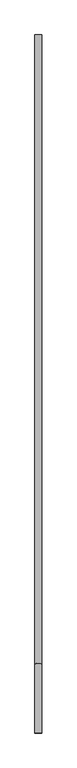
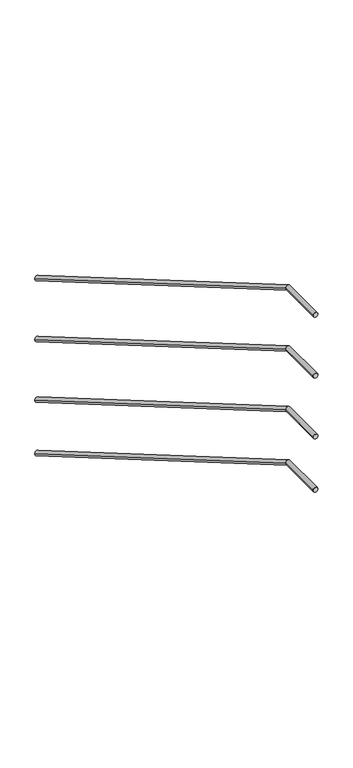
"""IFC4 building model written with IfcOpenShell, lengths in millimetres: railing geometry."""

from ifc_helpers import new_model, si_unit, frame, origin, place, context, project, spatial, circle_curve, ellipse_curve, source, transform, mapped, element, save
from ifc_brep_helpers import plane_surface, cylinder_surface, advanced_brep


def railing_58bcc5ab(model_context):
    return source(origin(), model_context, "Body", "AdvancedBrep", [
        advanced_brep(
        [(-1709.6, 15799.5208589, 8657.5963084), (-1739.6, 15799.5208589, 8657.5963084), (-1709.6, 13095.4656218, 10234.9618634), (-1739.6, 13095.4656218, 10234.9618634), (-1709.6, 12799.5208589, 10234.9618634), (-1739.6, 12799.5208589, 10234.9618634)],
        [
            (0, 1, ellipse_curve(frame((-1724.6, 15799.5208589, 8657.5963084), z_axis=(0.0, 1.0, 0.0), x_axis=(0.0, 0.0, -1.0)), 17.365555, 15.0)),
            (1, 0, ellipse_curve(frame((-1724.6, 15799.5208589, 8657.5963084), z_axis=(0.0, 1.0, 0.0), x_axis=(0.0, 0.0, -1.0)), 17.365555, 15.0)),
            (0, 2),
            (2, 3, ellipse_curve(frame((-1724.6, 13095.4656218, 10234.9618634), z_axis=(0.0, 0.9653442134540492, -0.2609799792144661), x_axis=(0.0, -0.26097997921446625, -0.9653442134540491)), 15.5384989, 15.0)),
            (3, 1),
            (3, 2, ellipse_curve(frame((-1724.6, 13095.4656218, 10234.9618634), z_axis=(0.0, 0.9653442134540492, -0.2609799792144661), x_axis=(0.0, -0.26097997921446625, -0.9653442134540491)), 15.5384989, 15.0)),
            (4, 5, circle_curve(frame((-1724.6, 12799.5208589, 10234.9618634), z_axis=(0.0, -1.0, 0.0), x_axis=(-1.0, 0.0, 0.0)), 15.0)),
            (5, 4, circle_curve(frame((-1724.6, 12799.5208589, 10234.9618634), z_axis=(0.0, -1.0, 0.0), x_axis=(-1.0, 0.0, 0.0)), 15.0)),
            (2, 4),
            (5, 3),
        ],
        [
            plane_surface(frame((-1724.6, 15799.5208589, 8674.9618634), z_axis=(0.0, 1.0, 0.0), x_axis=(0.0, 0.0, -1.0))),
            cylinder_surface(frame((-1724.6, 15791.9627935, 8662.0051799), z_axis=(0.0, 0.8637789008984337, -0.5038710255240858), x_axis=(-1.0, 0.0, 0.0)), 15.0),
            plane_surface(frame((-1724.6, 12799.5208589, 10249.9618634), z_axis=(0.0, -1.0, 0.0), x_axis=(0.0, 0.0, -1.0))),
            cylinder_surface(frame((-1724.6, 13099.5208589, 10234.9618634), z_axis=(0.0, 1.0, 0.0), x_axis=(-1.0, 0.0, 0.0)), 15.0),
        ],
        [
            (0, [[1, 2]]),
            (1, [[-1, 3, 4, 5]]),
            (1, [[-2, -5, 6, -3]]),
            (2, [[7, 8]]),
            (3, [[-4, 9, -8, 10]]),
            (3, [[-6, -10, -7, -9]]),
        ],
    ),
        advanced_brep(
        [(-1709.6, 15799.5208589, 7857.5963084), (-1739.6, 15799.5208589, 7857.5963084), (-1709.6, 13095.4656218, 9434.9618634), (-1739.6, 13095.4656218, 9434.9618634), (-1709.6, 12799.5208589, 9434.9618634), (-1739.6, 12799.5208589, 9434.9618634)],
        [
            (0, 1, ellipse_curve(frame((-1724.6, 15799.5208589, 7857.5963084), z_axis=(0.0, 1.0, 0.0), x_axis=(0.0, 0.0, -1.0)), 17.365555, 15.0)),
            (1, 0, ellipse_curve(frame((-1724.6, 15799.5208589, 7857.5963084), z_axis=(0.0, 1.0, 0.0), x_axis=(0.0, 0.0, -1.0)), 17.365555, 15.0)),
            (0, 2),
            (2, 3, ellipse_curve(frame((-1724.6, 13095.4656218, 9434.9618634), z_axis=(0.0, 0.9653442134540492, -0.2609799792144661), x_axis=(0.0, -0.26097997921446625, -0.9653442134540491)), 15.5384989, 15.0)),
            (3, 1),
            (3, 2, ellipse_curve(frame((-1724.6, 13095.4656218, 9434.9618634), z_axis=(0.0, 0.9653442134540492, -0.2609799792144661), x_axis=(0.0, -0.26097997921446625, -0.9653442134540491)), 15.5384989, 15.0)),
            (4, 5, circle_curve(frame((-1724.6, 12799.5208589, 9434.9618634), z_axis=(0.0, -1.0, 0.0), x_axis=(-1.0, 0.0, 0.0)), 15.0)),
            (5, 4, circle_curve(frame((-1724.6, 12799.5208589, 9434.9618634), z_axis=(0.0, -1.0, 0.0), x_axis=(-1.0, 0.0, 0.0)), 15.0)),
            (2, 4),
            (5, 3),
        ],
        [
            plane_surface(frame((-1724.6, 15799.5208589, 7874.9618634), z_axis=(0.0, 1.0, 0.0), x_axis=(0.0, 0.0, -1.0))),
            cylinder_surface(frame((-1724.6, 15791.9627935, 7862.0051799), z_axis=(0.0, 0.8637789008984337, -0.5038710255240858), x_axis=(-1.0, 0.0, 0.0)), 15.0),
            plane_surface(frame((-1724.6, 12799.5208589, 9449.9618634), z_axis=(0.0, -1.0, 0.0), x_axis=(0.0, 0.0, -1.0))),
            cylinder_surface(frame((-1724.6, 13099.5208589, 9434.9618634), z_axis=(0.0, 1.0, 0.0), x_axis=(-1.0, 0.0, 0.0)), 15.0),
        ],
        [
            (0, [[1, 2]]),
            (1, [[-1, 3, 4, 5]]),
            (1, [[-2, -5, 6, -3]]),
            (2, [[7, 8]]),
            (3, [[-4, 9, -8, 10]]),
            (3, [[-6, -10, -7, -9]]),
        ],
    ),
        advanced_brep(
        [(-1709.6, 15799.5208589, 8257.5963084), (-1739.6, 15799.5208589, 8257.5963084), (-1709.6, 13095.4656218, 9834.9618634), (-1739.6, 13095.4656218, 9834.9618634), (-1709.6, 12799.5208589, 9834.9618634), (-1739.6, 12799.5208589, 9834.9618634)],
        [
            (0, 1, ellipse_curve(frame((-1724.6, 15799.5208589, 8257.5963084), z_axis=(0.0, 1.0, 0.0), x_axis=(0.0, 0.0, -1.0)), 17.365555, 15.0)),
            (1, 0, ellipse_curve(frame((-1724.6, 15799.5208589, 8257.5963084), z_axis=(0.0, 1.0, 0.0), x_axis=(0.0, 0.0, -1.0)), 17.365555, 15.0)),
            (0, 2),
            (2, 3, ellipse_curve(frame((-1724.6, 13095.4656218, 9834.9618634), z_axis=(0.0, 0.9653442134540492, -0.2609799792144661), x_axis=(0.0, -0.26097997921446625, -0.9653442134540491)), 15.5384989, 15.0)),
            (3, 1),
            (3, 2, ellipse_curve(frame((-1724.6, 13095.4656218, 9834.9618634), z_axis=(0.0, 0.9653442134540492, -0.2609799792144661), x_axis=(0.0, -0.26097997921446625, -0.9653442134540491)), 15.5384989, 15.0)),
            (4, 5, circle_curve(frame((-1724.6, 12799.5208589, 9834.9618634), z_axis=(0.0, -1.0, 0.0), x_axis=(-1.0, 0.0, 0.0)), 15.0)),
            (5, 4, circle_curve(frame((-1724.6, 12799.5208589, 9834.9618634), z_axis=(0.0, -1.0, 0.0), x_axis=(-1.0, 0.0, 0.0)), 15.0)),
            (2, 4),
            (5, 3),
        ],
        [
            plane_surface(frame((-1724.6, 15799.5208589, 8274.9618634), z_axis=(0.0, 1.0, 0.0), x_axis=(0.0, 0.0, -1.0))),
            cylinder_surface(frame((-1724.6, 15791.9627935, 8262.0051799), z_axis=(0.0, 0.8637789008984337, -0.5038710255240858), x_axis=(-1.0, 0.0, 0.0)), 15.0),
            plane_surface(frame((-1724.6, 12799.5208589, 9849.9618634), z_axis=(0.0, -1.0, 0.0), x_axis=(0.0, 0.0, -1.0))),
            cylinder_surface(frame((-1724.6, 13099.5208589, 9834.9618634), z_axis=(0.0, 1.0, 0.0), x_axis=(-1.0, 0.0, 0.0)), 15.0),
        ],
        [
            (0, [[1, 2]]),
            (1, [[-1, 3, 4, 5]]),
            (1, [[-2, -5, 6, -3]]),
            (2, [[7, 8]]),
            (3, [[-4, 9, -8, 10]]),
            (3, [[-6, -10, -7, -9]]),
        ],
    ),
        advanced_brep(
        [(-1709.6, 15799.5208589, 7507.5963084), (-1739.6, 15799.5208589, 7507.5963084), (-1709.6, 13095.4656218, 9084.9618634), (-1739.6, 13095.4656218, 9084.9618634), (-1709.6, 12799.5208589, 9084.9618634), (-1739.6, 12799.5208589, 9084.9618634)],
        [
            (0, 1, ellipse_curve(frame((-1724.6, 15799.5208589, 7507.5963084), z_axis=(0.0, 1.0, 0.0), x_axis=(0.0, 0.0, -1.0)), 17.365555, 15.0)),
            (1, 0, ellipse_curve(frame((-1724.6, 15799.5208589, 7507.5963084), z_axis=(0.0, 1.0, 0.0), x_axis=(0.0, 0.0, -1.0)), 17.365555, 15.0)),
            (0, 2),
            (2, 3, ellipse_curve(frame((-1724.6, 13095.4656218, 9084.9618634), z_axis=(0.0, 0.9653442134540492, -0.2609799792144661), x_axis=(0.0, -0.26097997921446625, -0.9653442134540491)), 15.5384989, 15.0)),
            (3, 1),
            (3, 2, ellipse_curve(frame((-1724.6, 13095.4656218, 9084.9618634), z_axis=(0.0, 0.9653442134540492, -0.2609799792144661), x_axis=(0.0, -0.26097997921446625, -0.9653442134540491)), 15.5384989, 15.0)),
            (4, 5, circle_curve(frame((-1724.6, 12799.5208589, 9084.9618634), z_axis=(0.0, -1.0, 0.0), x_axis=(-1.0, 0.0, 0.0)), 15.0)),
            (5, 4, circle_curve(frame((-1724.6, 12799.5208589, 9084.9618634), z_axis=(0.0, -1.0, 0.0), x_axis=(-1.0, 0.0, 0.0)), 15.0)),
            (2, 4),
            (5, 3),
        ],
        [
            plane_surface(frame((-1724.6, 15799.5208589, 7524.9618634), z_axis=(0.0, 1.0, 0.0), x_axis=(0.0, 0.0, -1.0))),
            cylinder_surface(frame((-1724.6, 15791.9627935, 7512.0051799), z_axis=(0.0, 0.8637789008984337, -0.5038710255240858), x_axis=(-1.0, 0.0, 0.0)), 15.0),
            plane_surface(frame((-1724.6, 12799.5208589, 9099.9618634), z_axis=(0.0, -1.0, 0.0), x_axis=(0.0, 0.0, -1.0))),
            cylinder_surface(frame((-1724.6, 13099.5208589, 9084.9618634), z_axis=(0.0, 1.0, 0.0), x_axis=(-1.0, 0.0, 0.0)), 15.0),
        ],
        [
            (0, [[1, 2]]),
            (1, [[-1, 3, 4, 5]]),
            (1, [[-2, -5, 6, -3]]),
            (2, [[7, 8]]),
            (3, [[-4, 9, -8, 10]]),
            (3, [[-6, -10, -7, -9]]),
        ],
    ),
    ])


if __name__ == "__main__":
    model = new_model("IFC4")
    model_context = context("Model", 3, world=origin())
    ifc_project = project(units=[si_unit("LENGTHUNIT", "METRE", prefix="MILLI")], contexts=[model_context])
    site = spatial("IfcSite", under=ifc_project)
    building = spatial("IfcBuilding", under=site)
    placement = place(None, origin())
    railing_shape = railing_58bcc5ab(model_context)
    element("IfcRailing", 1, at=placement, inside=building, context=model_context, shape_type="MappedRepresentation", body=[
        mapped(railing_shape, transform((0.0, 0.0, 0.0), x_axis=(1.0, 0.0, 0.0), y_axis=(0.0, 1.0, 0.0), z_axis=(0.0, 0.0, 1.0))),
    ])
    save(model, "model.ifc")
